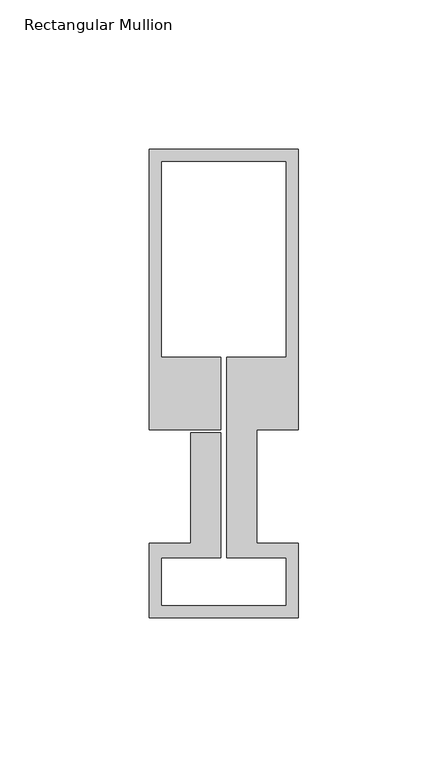
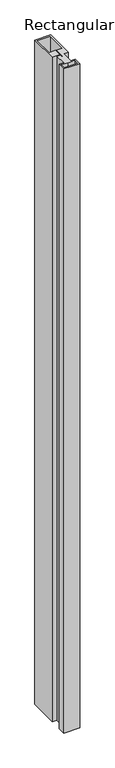
"""IFC4 building model written with IfcOpenShell, lengths in millimetres: member geometry, Rectangular Mullion : Schueco_FWS-50-SI_Mull_CovCap-20mm_Mull-85mm."""

from ifc_helpers import new_model, si_unit, frame, origin, place, context, project, spatial, polyline, outline, extrude, source, transform, mapped, element, save


def rectangular_mullion_93208227(model_context):
    return source(origin(), model_context, "Body", "SweptSolid", [
        extrude(outline(polyline([(0.0, 132.0), (0.0, 38.0), (-14.0, 38.0), (-14.0, -0.1), (0.0, -0.1), (0.0, -25.0), (-50.0, -25.0), (-50.0, -0.1), (-36.0, -0.1), (-36.0, 37.0), (-26.0, 37.0), (-26.0, -5.0), (-46.0, -5.0), (-46.0, -21.0), (-4.0, -21.0), (-4.0, -5.0), (-24.0, -5.0), (-24.0, 62.3), (-4.0, 62.3), (-4.0, 128.0), (-46.0, 128.0), (-46.0, 62.3), (-26.0, 62.3), (-26.0, 38.0), (-50.0, 38.0), (-50.0, 132.0), (0.0, 132.0)])), frame((0.0, 0.0, -2200.0), z_axis=(0.0, 0.0, 1.0), x_axis=(1.0, 0.0, 0.0)), (0.0, 0.0, 1.0), 2200.0),
    ])


if __name__ == "__main__":
    model = new_model("IFC4")
    model_context = context("Model", 3, world=origin())
    ifc_project = project(units=[si_unit("LENGTHUNIT", "METRE", prefix="MILLI")], contexts=[model_context])
    site = spatial("IfcSite", under=ifc_project)
    building = spatial("IfcBuilding", under=site)
    placement = place(None, origin())
    rectangular_mullion_shape = rectangular_mullion_93208227(model_context)
    element("IfcMember", 1, ObjectType="Rectangular Mullion : Schueco_FWS-50-SI_Mull_CovCap-20mm_Mull-85mm", at=placement, inside=building, context=model_context, shape_type="MappedRepresentation", body=[
        mapped(rectangular_mullion_shape, transform((0.0, 0.0, 0.0), x_axis=(1.0, 0.0, 0.0), y_axis=(0.0, 1.0, 0.0), z_axis=(0.0, 0.0, 1.0))),
    ])
    save(model, "model.ifc")

# Revit data of these elements
# Type "Rectangular Mullion : Schueco_FWS-50-SI_Mull_CovCap-20mm_Mull-85mm"
#   Model = "FWS 50.SI"
#   Manufacturer = "Schueco International KG"
#   Type Comments = "Mullion"
#   Schueco thermal insulation standard = "Suitable for passive houses"
#   Burglar resistance = "RC 3"
#   Thermal insulation = "to 0.70 W/(m²K)"
#   built-in parameter 1007322 = 0.515092 (stored number, unit not read)
#   built-in parameter 1007321 = 0.0360892 (stored number, unit not read)
#   built-in parameter 1007320 = 0.0360892 (stored number, unit not read)
# Element 1 (IfcMember, "Rectangular Mullion : Schueco_FWS-50-SI_Mull_CovCap-20mm_Mull-85mm")
#   Materials on its faces: "Alu"
# Materials
#   "Alu": class "Glas", colour RGB 140 140 140, transparency 0
